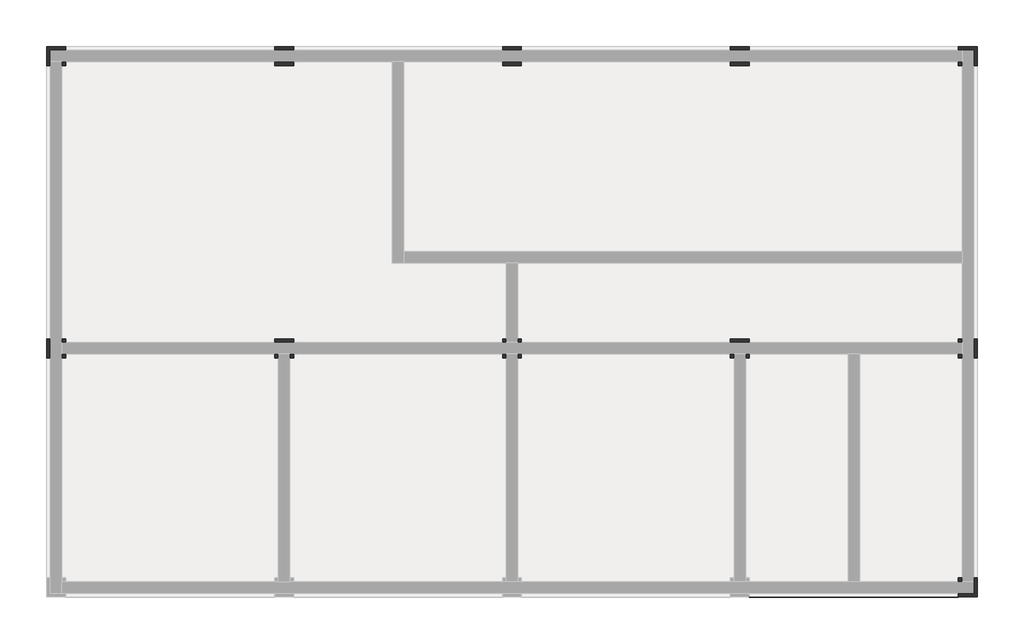
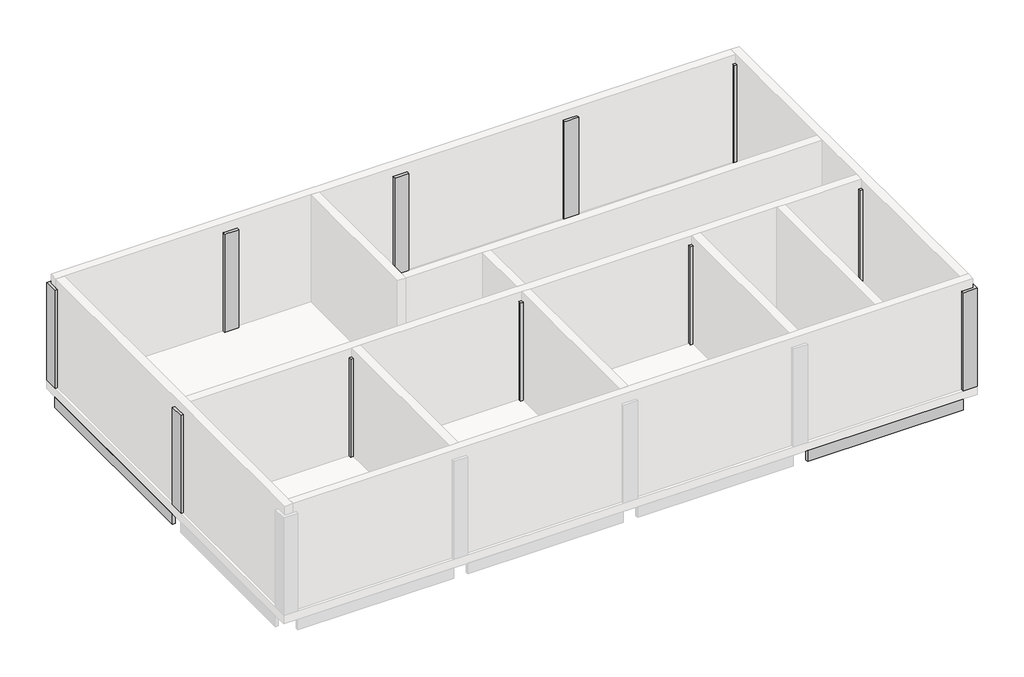
# One storey, part 2 of 2: 15 beams, 11 columns.
"""IFC4 building model written with IfcOpenShell, lengths in millimetres."""

from ifc_helpers import new_model, si_unit, frame, origin, place, context, project, spatial, polyline, outline, extrude, faceted_brep, element, save

model = new_model("IFC4")

# Units and contexts
model_context = context("Model", 3, world=origin())
ifc_project = project(units=[si_unit("LENGTHUNIT", "METRE", prefix="MILLI")], contexts=[model_context])

# Site, building, storey
site = spatial("IfcSite", under=ifc_project)
building = spatial("IfcBuilding", under=site)
storey = spatial("IfcBuildingStorey", under=building, Name="2nd FL GL+6,200", Elevation=6000.0)

# Beams
placement = place(None, origin())
element("IfcBeam", 1, ObjectType="RC Beam_Rectangular : 350 x 700mm", at=placement, inside=storey, context=model_context, shape_type="SweptSolid", body=[
    extrude(outline(polyline([(-18945.7273237, 9185.9763125), (-18845.7273237, 9185.9763125), (-18845.7273237, 1985.9763125), (-18945.7273237, 1985.9763125), (-18945.7273237, 9185.9763125)])), frame((0.0, 0.0, 5300.0), z_axis=(0.0, 0.0, 1.0), x_axis=(1.0, 0.0, 0.0)), (0.0, 0.0, 1.0), 400.0),
])
element("IfcBeam", 2, ObjectType="RC Beam_Rectangular : 350 x 700mm", at=placement, inside=storey, context=model_context, shape_type="SweptSolid", body=[
    extrude(outline(polyline([(-12870.7273237, 9185.9763125), (-12520.7273237, 9185.9763125), (-12520.7273237, 1985.9763125), (-12870.7273237, 1985.9763125), (-12870.7273237, 9185.9763125)])), frame((0.0, 0.0, 5300.0), z_axis=(0.0, 0.0, 1.0), x_axis=(1.0, 0.0, 0.0)), (0.0, 0.0, 1.0), 400.0),
])
element("IfcBeam", 3, ObjectType="RC Beam_Rectangular : 350 x 700mm", at=placement, inside=storey, context=model_context, shape_type="SweptSolid", body=[
    extrude(outline(polyline([(-6870.7273237, 9185.9763125), (-6520.7273237, 9185.9763125), (-6520.7273237, 1985.9763125), (-6870.7273237, 1985.9763125), (-6870.7273237, 9185.9763125)])), frame((0.0, 0.0, 5300.0), z_axis=(0.0, 0.0, 1.0), x_axis=(1.0, 0.0, 0.0)), (0.0, 0.0, 1.0), 400.0),
])
element("IfcBeam", 4, ObjectType="RC Beam_Rectangular : 350 x 700mm", at=placement, inside=storey, context=model_context, shape_type="SweptSolid", body=[
    extrude(outline(polyline([(-870.7273237, 9185.9763125), (-520.7273237, 9185.9763125), (-520.7273237, 1985.9763125), (-870.7273237, 1985.9763125), (-870.7273237, 9185.9763125)])), frame((0.0, 0.0, 5300.0), z_axis=(0.0, 0.0, 1.0), x_axis=(1.0, 0.0, 0.0)), (0.0, 0.0, 1.0), 400.0),
])
element("IfcBeam", 5, ObjectType="RC Beam_Rectangular : 350 x 700mm", at=placement, inside=storey, context=model_context, shape_type="SweptSolid", body=[
    extrude(outline(polyline([(5554.2726763, 1485.9763125), (5554.2726763, -4314.0236875), (5454.2726763, -4314.0236875), (5454.2726763, 1485.9763125), (5554.2726763, 1485.9763125)])), frame((0.0, 0.0, 5300.0), z_axis=(0.0, 0.0, 1.0), x_axis=(1.0, 0.0, 0.0)), (0.0, 0.0, 1.0), 400.0),
])
element("IfcBeam", 6, ObjectType="RC Beam_Rectangular : 350 x 700mm", at=placement, inside=storey, context=model_context, shape_type="SweptSolid", body=[
    extrude(outline(polyline([(5554.2726763, 9185.9763125), (5554.2726763, 1998.6763125), (5454.2726763, 1998.6763125), (5454.2726763, 9185.9763125), (5554.2726763, 9185.9763125)])), frame((0.0, 0.0, 5300.0), z_axis=(0.0, 0.0, 1.0), x_axis=(1.0, 0.0, 0.0)), (0.0, 0.0, 1.0), 400.0),
])
element("IfcBeam", 7, ObjectType="RC Beam_Rectangular : 350 x 700mm", at=placement, inside=storey, context=model_context, shape_type="SweptSolid", body=[
    extrude(outline(polyline([(-18445.7273237, 9685.9763125), (-12945.7273237, 9685.9763125), (-12945.7273237, 9585.9763125), (-18445.7273237, 9585.9763125), (-18445.7273237, 9685.9763125)])), frame((0.0, 0.0, 5300.0), z_axis=(0.0, 0.0, 1.0), x_axis=(1.0, 0.0, 0.0)), (0.0, 0.0, 1.0), 400.0),
])
element("IfcBeam", 8, ObjectType="RC Beam_Rectangular : 350 x 700mm", at=placement, inside=storey, context=model_context, shape_type="SweptSolid", body=[
    extrude(outline(polyline([(-12433.0273237, 9685.9763125), (-6945.7273237, 9685.9763125), (-6945.7273237, 9585.9763125), (-12433.0273237, 9585.9763125), (-12433.0273237, 9685.9763125)])), frame((0.0, 0.0, 5300.0), z_axis=(0.0, 0.0, 1.0), x_axis=(1.0, 0.0, 0.0)), (0.0, 0.0, 1.0), 400.0),
])
element("IfcBeam", 9, ObjectType="RC Beam_Rectangular : 350 x 700mm", at=placement, inside=storey, context=model_context, shape_type="SweptSolid", body=[
    extrude(outline(polyline([(-6433.0273237, 9685.9763125), (-945.7273237, 9685.9763125), (-945.7273237, 9585.9763125), (-6433.0273237, 9585.9763125), (-6433.0273237, 9685.9763125)])), frame((0.0, 0.0, 5300.0), z_axis=(0.0, 0.0, 1.0), x_axis=(1.0, 0.0, 0.0)), (0.0, 0.0, 1.0), 400.0),
])
element("IfcBeam", 10, ObjectType="RC Beam_Rectangular : 350 x 700mm", at=placement, inside=storey, context=model_context, shape_type="SweptSolid", body=[
    extrude(outline(polyline([(-433.0273237, 9685.9763125), (5054.2726763, 9685.9763125), (5054.2726763, 9585.9763125), (-433.0273237, 9585.9763125), (-433.0273237, 9685.9763125)])), frame((0.0, 0.0, 5300.0), z_axis=(0.0, 0.0, 1.0), x_axis=(1.0, 0.0, 0.0)), (0.0, 0.0, 1.0), 400.0),
])
element("IfcBeam", 11, ObjectType="RC Beam_Rectangular : 350 x 700mm", at=placement, inside=storey, context=model_context, shape_type="SweptSolid", body=[
    extrude(outline(polyline([(-12945.7273237, 1560.9763125), (-18445.7273237, 1560.9763125), (-18445.7273237, 1585.9763125), (-12945.7273237, 1585.9763125), (-12945.7273237, 1560.9763125)])), frame((0.0, 0.0, 5300.0), z_axis=(0.0, 0.0, 1.0), x_axis=(1.0, 0.0, 0.0)), (0.0, 0.0, 1.0), 400.0),
    extrude(outline(polyline([(-18445.7273237, 1910.9763125), (-12945.7273237, 1910.9763125), (-12945.7273237, 1885.9763125), (-18445.7273237, 1885.9763125), (-18445.7273237, 1910.9763125)])), frame((0.0, 0.0, 5300.0), z_axis=(0.0, 0.0, 1.0), x_axis=(1.0, 0.0, 0.0)), (0.0, 0.0, 1.0), 400.0),
])
element("IfcBeam", 12, ObjectType="RC Beam_Rectangular : 350 x 700mm", at=placement, inside=storey, context=model_context, shape_type="SweptSolid", body=[
    extrude(outline(polyline([(-6945.7273237, 1585.9763125), (-6945.7273237, 1560.9763125), (-12445.7273237, 1560.9763125), (-12445.7273237, 1585.9763125), (-6945.7273237, 1585.9763125)])), frame((0.0, 0.0, 5300.0), z_axis=(0.0, 0.0, 1.0), x_axis=(1.0, 0.0, 0.0)), (0.0, 0.0, 1.0), 400.0),
    extrude(outline(polyline([(-6945.7273237, 1910.9763125), (-6945.7273237, 1885.9763125), (-12445.7273237, 1885.9763125), (-12445.7273237, 1910.9763125), (-6945.7273237, 1910.9763125)])), frame((0.0, 0.0, 5300.0), z_axis=(0.0, 0.0, 1.0), x_axis=(1.0, 0.0, 0.0)), (0.0, 0.0, 1.0), 400.0),
])
element("IfcBeam", 13, ObjectType="RC Beam_Rectangular : 350 x 700mm", at=placement, inside=storey, context=model_context, shape_type="SweptSolid", body=[
    extrude(outline(polyline([(-945.7273237, 1585.9763125), (-945.7273237, 1560.9763125), (-6445.7273237, 1560.9763125), (-6445.7273237, 1585.9763125), (-945.7273237, 1585.9763125)])), frame((0.0, 0.0, 5300.0), z_axis=(0.0, 0.0, 1.0), x_axis=(1.0, 0.0, 0.0)), (0.0, 0.0, 1.0), 400.0),
    extrude(outline(polyline([(-945.7273237, 1910.9763125), (-945.7273237, 1885.9763125), (-6445.7273237, 1885.9763125), (-6445.7273237, 1910.9763125), (-945.7273237, 1910.9763125)])), frame((0.0, 0.0, 5300.0), z_axis=(0.0, 0.0, 1.0), x_axis=(1.0, 0.0, 0.0)), (0.0, 0.0, 1.0), 400.0),
])
element("IfcBeam", 14, ObjectType="RC Beam_Rectangular : 350 x 700mm", at=placement, inside=storey, context=model_context, shape_type="SweptSolid", body=[
    extrude(outline(polyline([(2154.2726763, 1585.9763125), (2154.2726763, 1560.9763125), (-445.7273237, 1560.9763125), (-445.7273237, 1585.9763125), (2154.2726763, 1585.9763125)])), frame((0.0, 0.0, 5300.0), z_axis=(0.0, 0.0, 1.0), x_axis=(1.0, 0.0, 0.0)), (0.0, 0.0, 1.0), 400.0),
    extrude(outline(polyline([(5054.2726763, 1910.9763125), (5054.2726763, 1885.9763125), (-445.7273237, 1885.9763125), (-445.7273237, 1910.9763125), (5054.2726763, 1910.9763125)])), frame((0.0, 0.0, 5300.0), z_axis=(0.0, 0.0, 1.0), x_axis=(1.0, 0.0, 0.0)), (0.0, 0.0, 1.0), 400.0),
    extrude(outline(polyline([(5054.2726763, 1585.9763125), (5054.2726763, 1560.9763125), (2454.2726763, 1560.9763125), (2454.2726763, 1585.9763125), (5054.2726763, 1585.9763125)])), frame((0.0, 0.0, 5300.0), z_axis=(0.0, 0.0, 1.0), x_axis=(1.0, 0.0, 0.0)), (0.0, 0.0, 1.0), 400.0),
])
element("IfcBeam", 15, ObjectType="RC Beam_Rectangular : 350 x 700mm", at=placement, inside=storey, context=model_context, shape_type="SweptSolid", body=[
    extrude(outline(polyline([(5054.2726763, -4714.0236875), (5054.2726763, -4814.0236875), (-445.7273237, -4814.0236875), (-445.7273237, -4714.0236875), (5054.2726763, -4714.0236875)])), frame((0.0, 0.0, 5300.0), z_axis=(0.0, 0.0, 1.0), x_axis=(1.0, 0.0, 0.0)), (0.0, 0.0, 1.0), 400.0),
])

# Columns
element("IfcColumn", 16, ObjectType="RC_Column_Rectangular : 500 x 500mm", at=placement, inside=storey, context=model_context, shape_type="Brep", body=[
    faceted_brep([(-18945.7273237, 9185.9763125, 6000.0), (-18945.7273237, 9685.9763125, 6000.0), (-18445.7273237, 9685.9763125, 6000.0), (-18445.7273237, 9585.9763125, 6000.0), (-18845.7273237, 9585.9763125, 6000.0), (-18845.7273237, 9285.9763125, 6000.0), (-18845.7273237, 9185.9763125, 6000.0), (-18945.7273237, 9685.9763125, 9667.0), (-18445.7273237, 9685.9763125, 9667.0), (-18445.7273237, 9685.9763125, 9300.0), (-18945.7273237, 9185.9763125, 9300.0), (-18945.7273237, 9185.9763125, 9667.0), (-18845.7273237, 9185.9763125, 9300.0), (-18845.7273237, 9185.9763125, 9667.0), (-18445.7273237, 9585.9763125, 9667.0), (-18445.7273237, 9585.9763125, 9300.0), (-18845.7273237, 9585.9763125, 9667.0)], [[[0, 1, 2, 3, 4, 5, 6]], [[2, 1, 7, 8, 9]], [[1, 0, 10, 11, 7]], [[11, 10, 0, 6, 12, 13]], [[2, 9, 8, 14, 15, 3]], [[8, 7, 11, 13, 16, 14]], [[16, 4, 3, 15, 14]], [[4, 16, 13, 12, 6, 5]]]),
    faceted_brep([(-18445.7273237, 9285.9763125, 9667.0), (-18445.7273237, 9285.9763125, 6000.0), (-18545.7273237, 9285.9763125, 6000.0), (-18545.7273237, 9285.9763125, 9667.0), (-18445.7273237, 9185.9763125, 9667.0), (-18445.7273237, 9185.9763125, 6000.0), (-18545.7273237, 9185.9763125, 6000.0), (-18545.7273237, 9185.9763125, 9667.0)], [[[0, 1, 2, 3]], [[4, 5, 1, 0]], [[2, 6, 7, 3]], [[1, 5, 6, 2]], [[5, 4, 7, 6]], [[4, 0, 3, 7]]]),
])
element("IfcColumn", 17, ObjectType="RC_Column_Rectangular : 500 x 500mm", at=placement, inside=storey, context=model_context, shape_type="Brep", body=[
    faceted_brep([(-18945.7273237, 1485.9763125, 6000.0), (-18945.7273237, 1985.9763125, 6000.0), (-18845.7273237, 1985.9763125, 6000.0), (-18845.7273237, 1485.9763125, 6000.0), (-18945.7273237, 1485.9763125, 9300.0), (-18945.7273237, 1485.9763125, 9667.0), (-18945.7273237, 1985.9763125, 9667.0), (-18845.7273237, 1485.9763125, 9300.0), (-18845.7273237, 1485.9763125, 9667.0), (-18845.7273237, 1985.9763125, 9667.0)], [[[0, 1, 2, 3]], [[1, 0, 4, 5, 6]], [[5, 4, 0, 3, 7, 8]], [[6, 5, 8, 9]], [[3, 2, 9, 8, 7]], [[1, 6, 9, 2]]]),
    faceted_brep([(-18445.7273237, 1985.9763125, 9667.0), (-18445.7273237, 1985.9763125, 6000.0), (-18545.7273237, 1985.9763125, 6000.0), (-18545.7273237, 1985.9763125, 9667.0), (-18445.7273237, 1910.9763125, 9667.0), (-18445.7273237, 1885.9763125, 9667.0), (-18445.7273237, 1885.9763125, 9300.0), (-18445.7273237, 1885.9763125, 6000.0), (-18545.7273237, 1885.9763125, 6000.0), (-18545.7273237, 1885.9763125, 9667.0)], [[[0, 1, 2, 3]], [[1, 0, 4, 5, 6, 7]], [[2, 1, 7, 8]], [[0, 3, 9, 5, 4]], [[7, 6, 5, 9, 8]], [[3, 2, 8, 9]]]),
    faceted_brep([(-18545.7273237, 1485.9763125, 6000.0), (-18545.7273237, 1485.9763125, 9667.0), (-18545.7273237, 1585.9763125, 9667.0), (-18545.7273237, 1585.9763125, 6000.0), (-18445.7273237, 1485.9763125, 6000.0), (-18445.7273237, 1485.9763125, 9667.0), (-18445.7273237, 1585.9763125, 9667.0), (-18445.7273237, 1585.9763125, 9300.0), (-18445.7273237, 1585.9763125, 6000.0), (-18445.7273237, 1560.9763125, 9667.0)], [[[0, 1, 2, 3]], [[4, 5, 1, 0]], [[6, 7, 8, 3, 2]], [[5, 4, 8, 7, 6, 9]], [[4, 0, 3, 8]], [[1, 5, 9, 6, 2]]]),
])
element("IfcColumn", 18, ObjectType="RC_Column_Rectangular : 500 x 500mm", at=placement, inside=storey, context=model_context, shape_type="Brep", body=[
    faceted_brep([(-12945.7273237, 9685.9763125, 6000.0), (-12445.7273237, 9685.9763125, 6000.0), (-12445.7273237, 9585.9763125, 6000.0), (-12945.7273237, 9585.9763125, 6000.0), (-12945.7273237, 9685.9763125, 9300.0), (-12945.7273237, 9685.9763125, 9667.0), (-12445.7273237, 9685.9763125, 9667.0), (-12445.7273237, 9685.9763125, 9300.0), (-12945.7273237, 9585.9763125, 9300.0), (-12945.7273237, 9585.9763125, 9667.0), (-12445.7273237, 9585.9763125, 9667.0), (-12445.7273237, 9585.9763125, 9300.0)], [[[0, 1, 2, 3]], [[1, 0, 4, 5, 6, 7]], [[5, 4, 0, 3, 8, 9]], [[1, 7, 6, 10, 11, 2]], [[6, 5, 9, 10]], [[3, 2, 11, 10, 9, 8]]]),
    faceted_brep([(-12945.7273237, 9185.9763125, 6000.0), (-12445.7273237, 9185.9763125, 6000.0), (-12445.7273237, 9185.9763125, 9667.0), (-12520.7273237, 9185.9763125, 9667.0), (-12870.7273237, 9185.9763125, 9667.0), (-12945.7273237, 9185.9763125, 9667.0), (-12445.7273237, 9285.9763125, 6000.0), (-12945.7273237, 9285.9763125, 6000.0), (-12945.7273237, 9285.9763125, 9667.0), (-12445.7273237, 9285.9763125, 9667.0)], [[[0, 1, 2, 3, 4, 5]], [[6, 7, 8, 9]], [[1, 0, 7, 6]], [[0, 5, 8, 7]], [[2, 1, 6, 9]], [[5, 4, 3, 2, 9, 8]]]),
])
element("IfcColumn", 19, ObjectType="RC_Column_Rectangular : 500 x 500mm", at=placement, inside=storey, context=model_context, shape_type="Brep", body=[
    faceted_brep([(-12945.7273237, 1985.9763125, 6000.0), (-12445.7273237, 1985.9763125, 6000.0), (-12445.7273237, 1885.9763125, 6000.0), (-12945.7273237, 1885.9763125, 6000.0), (-12945.7273237, 1985.9763125, 9667.0), (-12870.7273237, 1985.9763125, 9667.0), (-12520.7273237, 1985.9763125, 9667.0), (-12445.7273237, 1985.9763125, 9667.0), (-12945.7273237, 1885.9763125, 9300.0), (-12945.7273237, 1885.9763125, 9667.0), (-12945.7273237, 1910.9763125, 9667.0), (-12445.7273237, 1910.9763125, 9667.0), (-12445.7273237, 1885.9763125, 9667.0), (-12445.7273237, 1885.9763125, 9300.0)], [[[0, 1, 2, 3]], [[1, 0, 4, 5, 6, 7]], [[4, 0, 3, 8, 9, 10]], [[1, 7, 11, 12, 13, 2]], [[7, 6, 5, 4, 10, 9, 12, 11]], [[3, 2, 13, 12, 9, 8]]]),
    faceted_brep([(-12945.7273237, 1485.9763125, 9667.0), (-12945.7273237, 1485.9763125, 6000.0), (-12845.7273237, 1485.9763125, 6000.0), (-12845.7273237, 1485.9763125, 9300.0), (-12845.7273237, 1485.9763125, 9667.0), (-12870.7273237, 1485.9763125, 9667.0), (-12945.7273237, 1585.9763125, 6000.0), (-12945.7273237, 1585.9763125, 9300.0), (-12945.7273237, 1585.9763125, 9667.0), (-12845.7273237, 1585.9763125, 9667.0), (-12845.7273237, 1585.9763125, 6000.0), (-12945.7273237, 1560.9763125, 9667.0)], [[[0, 1, 2, 3, 4, 5]], [[6, 7, 8, 9, 10]], [[1, 6, 10, 2]], [[1, 0, 11, 8, 7, 6]], [[8, 11, 0, 5, 4, 9]], [[4, 3, 2, 10, 9]]]),
    faceted_brep([(-12445.7273237, 1485.9763125, 9667.0), (-12445.7273237, 1485.9763125, 6000.0), (-12445.7273237, 1585.9763125, 6000.0), (-12445.7273237, 1585.9763125, 9300.0), (-12445.7273237, 1585.9763125, 9667.0), (-12445.7273237, 1560.9763125, 9667.0), (-12545.7273237, 1485.9763125, 6000.0), (-12545.7273237, 1485.9763125, 9300.0), (-12545.7273237, 1485.9763125, 9667.0), (-12545.7273237, 1585.9763125, 9667.0), (-12545.7273237, 1585.9763125, 6000.0), (-12520.7273237, 1485.9763125, 9667.0)], [[[0, 1, 2, 3, 4, 5]], [[6, 7, 8, 9, 10]], [[1, 0, 11, 8, 7, 6]], [[4, 3, 2, 10, 9]], [[2, 1, 6, 10]], [[0, 5, 4, 9, 8, 11]]]),
])
element("IfcColumn", 20, ObjectType="RC_Column_Rectangular : 500 x 500mm", at=placement, inside=storey, context=model_context, shape_type="Brep", body=[
    faceted_brep([(-6945.7273237, 9685.9763125, 6000.0), (-6445.7273237, 9685.9763125, 6000.0), (-6445.7273237, 9585.9763125, 6000.0), (-6945.7273237, 9585.9763125, 6000.0), (-6945.7273237, 9685.9763125, 9300.0), (-6945.7273237, 9685.9763125, 9667.0), (-6445.7273237, 9685.9763125, 9667.0), (-6445.7273237, 9685.9763125, 9300.0), (-6945.7273237, 9585.9763125, 9300.0), (-6945.7273237, 9585.9763125, 9667.0), (-6445.7273237, 9585.9763125, 9667.0), (-6445.7273237, 9585.9763125, 9300.0)], [[[0, 1, 2, 3]], [[1, 0, 4, 5, 6, 7]], [[5, 4, 0, 3, 8, 9]], [[1, 7, 6, 10, 11, 2]], [[6, 5, 9, 10]], [[3, 2, 11, 10, 9, 8]]]),
    faceted_brep([(-6945.7273237, 9185.9763125, 6000.0), (-6445.7273237, 9185.9763125, 6000.0), (-6445.7273237, 9185.9763125, 9667.0), (-6520.7273237, 9185.9763125, 9667.0), (-6870.7273237, 9185.9763125, 9667.0), (-6945.7273237, 9185.9763125, 9667.0), (-6445.7273237, 9285.9763125, 6000.0), (-6945.7273237, 9285.9763125, 6000.0), (-6945.7273237, 9285.9763125, 9667.0), (-6445.7273237, 9285.9763125, 9667.0)], [[[0, 1, 2, 3, 4, 5]], [[6, 7, 8, 9]], [[1, 0, 7, 6]], [[0, 5, 8, 7]], [[2, 1, 6, 9]], [[5, 4, 3, 2, 9, 8]]]),
])
element("IfcColumn", 21, ObjectType="RC_Column_Rectangular : 500 x 500mm", at=placement, inside=storey, context=model_context, shape_type="Brep", body=[
    faceted_brep([(-6945.7273237, 1885.9763125, 6000.0), (-6945.7273237, 1985.9763125, 6000.0), (-6845.7273237, 1985.9763125, 6000.0), (-6845.7273237, 1885.9763125, 6000.0), (-6945.7273237, 1985.9763125, 9667.0), (-6945.7273237, 1885.9763125, 9300.0), (-6945.7273237, 1885.9763125, 9667.0), (-6945.7273237, 1910.9763125, 9667.0), (-6845.7273237, 1885.9763125, 9667.0), (-6845.7273237, 1985.9763125, 9667.0), (-6870.7273237, 1985.9763125, 9667.0), (-6845.7273237, 1985.9763125, 9300.0)], [[[0, 1, 2, 3]], [[4, 1, 0, 5, 6, 7]], [[4, 7, 6, 8, 9, 10]], [[3, 2, 11, 9, 8]], [[1, 4, 10, 9, 11, 2]], [[6, 5, 0, 3, 8]]]),
    faceted_brep([(-6445.7273237, 1985.9763125, 9667.0), (-6445.7273237, 1985.9763125, 6000.0), (-6545.7273237, 1985.9763125, 6000.0), (-6545.7273237, 1985.9763125, 9300.0), (-6545.7273237, 1985.9763125, 9667.0), (-6520.7273237, 1985.9763125, 9667.0), (-6445.7273237, 1910.9763125, 9667.0), (-6445.7273237, 1885.9763125, 9667.0), (-6445.7273237, 1885.9763125, 9300.0), (-6445.7273237, 1885.9763125, 6000.0), (-6545.7273237, 1885.9763125, 9667.0), (-6545.7273237, 1885.9763125, 6000.0)], [[[0, 1, 2, 3, 4, 5]], [[1, 0, 6, 7, 8, 9]], [[9, 8, 7, 10, 11]], [[2, 11, 10, 4, 3]], [[1, 9, 11, 2]], [[7, 6, 0, 5, 4, 10]]]),
    faceted_brep([(-6945.7273237, 1485.9763125, 9667.0), (-6945.7273237, 1485.9763125, 6000.0), (-6845.7273237, 1485.9763125, 6000.0), (-6845.7273237, 1485.9763125, 9300.0), (-6845.7273237, 1485.9763125, 9667.0), (-6870.7273237, 1485.9763125, 9667.0), (-6945.7273237, 1585.9763125, 6000.0), (-6945.7273237, 1585.9763125, 9300.0), (-6945.7273237, 1585.9763125, 9667.0), (-6845.7273237, 1585.9763125, 9667.0), (-6845.7273237, 1585.9763125, 6000.0), (-6945.7273237, 1560.9763125, 9667.0)], [[[0, 1, 2, 3, 4, 5]], [[6, 7, 8, 9, 10]], [[1, 6, 10, 2]], [[1, 0, 11, 8, 7, 6]], [[8, 11, 0, 5, 4, 9]], [[4, 3, 2, 10, 9]]]),
    faceted_brep([(-6445.7273237, 1485.9763125, 9667.0), (-6445.7273237, 1485.9763125, 6000.0), (-6445.7273237, 1585.9763125, 6000.0), (-6445.7273237, 1585.9763125, 9300.0), (-6445.7273237, 1585.9763125, 9667.0), (-6445.7273237, 1560.9763125, 9667.0), (-6545.7273237, 1485.9763125, 6000.0), (-6545.7273237, 1485.9763125, 9300.0), (-6545.7273237, 1485.9763125, 9667.0), (-6545.7273237, 1585.9763125, 9667.0), (-6545.7273237, 1585.9763125, 6000.0), (-6520.7273237, 1485.9763125, 9667.0)], [[[0, 1, 2, 3, 4, 5]], [[6, 7, 8, 9, 10]], [[1, 0, 11, 8, 7, 6]], [[4, 3, 2, 10, 9]], [[2, 1, 6, 10]], [[0, 5, 4, 9, 8, 11]]]),
])
element("IfcColumn", 22, ObjectType="RC_Column_Rectangular : 500 x 500mm", at=placement, inside=storey, context=model_context, shape_type="Brep", body=[
    faceted_brep([(-945.7273237, 9685.9763125, 6000.0), (-445.7273237, 9685.9763125, 6000.0), (-445.7273237, 9585.9763125, 6000.0), (-945.7273237, 9585.9763125, 6000.0), (-945.7273237, 9685.9763125, 9300.0), (-945.7273237, 9685.9763125, 9667.0), (-445.7273237, 9685.9763125, 9667.0), (-445.7273237, 9685.9763125, 9300.0), (-945.7273237, 9585.9763125, 9300.0), (-945.7273237, 9585.9763125, 9667.0), (-445.7273237, 9585.9763125, 9667.0), (-445.7273237, 9585.9763125, 9300.0)], [[[0, 1, 2, 3]], [[1, 0, 4, 5, 6, 7]], [[5, 4, 0, 3, 8, 9]], [[1, 7, 6, 10, 11, 2]], [[6, 5, 9, 10]], [[3, 2, 11, 10, 9, 8]]]),
    faceted_brep([(-945.7273237, 9185.9763125, 6000.0), (-445.7273237, 9185.9763125, 6000.0), (-445.7273237, 9185.9763125, 9667.0), (-520.7273237, 9185.9763125, 9667.0), (-870.7273237, 9185.9763125, 9667.0), (-945.7273237, 9185.9763125, 9667.0), (-445.7273237, 9285.9763125, 6000.0), (-945.7273237, 9285.9763125, 6000.0), (-945.7273237, 9285.9763125, 9667.0), (-445.7273237, 9285.9763125, 9667.0)], [[[0, 1, 2, 3, 4, 5]], [[6, 7, 8, 9]], [[1, 0, 7, 6]], [[0, 5, 8, 7]], [[2, 1, 6, 9]], [[5, 4, 3, 2, 9, 8]]]),
])
element("IfcColumn", 23, ObjectType="RC_Column_Rectangular : 500 x 500mm", at=placement, inside=storey, context=model_context, shape_type="Brep", body=[
    faceted_brep([(-945.7273237, 1985.9763125, 6000.0), (-445.7273237, 1985.9763125, 6000.0), (-445.7273237, 1885.9763125, 6000.0), (-945.7273237, 1885.9763125, 6000.0), (-945.7273237, 1985.9763125, 9667.0), (-870.7273237, 1985.9763125, 9667.0), (-520.7273237, 1985.9763125, 9667.0), (-445.7273237, 1985.9763125, 9667.0), (-945.7273237, 1885.9763125, 9300.0), (-945.7273237, 1885.9763125, 9667.0), (-945.7273237, 1910.9763125, 9667.0), (-445.7273237, 1910.9763125, 9667.0), (-445.7273237, 1885.9763125, 9667.0), (-445.7273237, 1885.9763125, 9300.0)], [[[0, 1, 2, 3]], [[1, 0, 4, 5, 6, 7]], [[4, 0, 3, 8, 9, 10]], [[1, 7, 11, 12, 13, 2]], [[7, 6, 5, 4, 10, 9, 12, 11]], [[3, 2, 13, 12, 9, 8]]]),
    faceted_brep([(-945.7273237, 1485.9763125, 9667.0), (-945.7273237, 1485.9763125, 6000.0), (-845.7273237, 1485.9763125, 6000.0), (-845.7273237, 1485.9763125, 9300.0), (-845.7273237, 1485.9763125, 9667.0), (-870.7273237, 1485.9763125, 9667.0), (-945.7273237, 1585.9763125, 6000.0), (-945.7273237, 1585.9763125, 9300.0), (-945.7273237, 1585.9763125, 9667.0), (-845.7273237, 1585.9763125, 9667.0), (-845.7273237, 1585.9763125, 6000.0), (-945.7273237, 1560.9763125, 9667.0)], [[[0, 1, 2, 3, 4, 5]], [[6, 7, 8, 9, 10]], [[1, 6, 10, 2]], [[1, 0, 11, 8, 7, 6]], [[8, 11, 0, 5, 4, 9]], [[4, 3, 2, 10, 9]]]),
    faceted_brep([(-445.7273237, 1485.9763125, 9667.0), (-445.7273237, 1485.9763125, 6000.0), (-445.7273237, 1585.9763125, 6000.0), (-445.7273237, 1585.9763125, 9300.0), (-445.7273237, 1585.9763125, 9667.0), (-445.7273237, 1560.9763125, 9667.0), (-545.7273237, 1485.9763125, 6000.0), (-545.7273237, 1485.9763125, 9300.0), (-545.7273237, 1485.9763125, 9667.0), (-545.7273237, 1585.9763125, 9667.0), (-545.7273237, 1585.9763125, 6000.0), (-520.7273237, 1485.9763125, 9667.0)], [[[0, 1, 2, 3, 4, 5]], [[6, 7, 8, 9, 10]], [[1, 0, 11, 8, 7, 6]], [[4, 3, 2, 10, 9]], [[2, 1, 6, 10]], [[0, 5, 4, 9, 8, 11]]]),
])
element("IfcColumn", 24, ObjectType="RC_Column_Rectangular : 500 x 500mm", at=placement, inside=storey, context=model_context, shape_type="Brep", body=[
    faceted_brep([(5054.2726763, 9185.9763125, 6000.0), (5054.2726763, 9285.9763125, 6000.0), (5154.2726763, 9285.9763125, 6000.0), (5154.2726763, 9185.9763125, 6000.0), (5054.2726763, 9185.9763125, 9667.0), (5154.2726763, 9185.9763125, 9667.0), (5054.2726763, 9285.9763125, 9667.0), (5154.2726763, 9285.9763125, 9667.0)], [[[0, 1, 2, 3]], [[4, 0, 3, 5]], [[6, 4, 5, 7]], [[2, 1, 6, 7]], [[0, 4, 6, 1]], [[3, 2, 7, 5]]]),
    faceted_brep([(5554.2726763, 9685.9763125, 6000.0), (5054.2726763, 9685.9763125, 6000.0), (5054.2726763, 9685.9763125, 9300.0), (5054.2726763, 9685.9763125, 9667.0), (5554.2726763, 9685.9763125, 9667.0), (5054.2726763, 9585.9763125, 6000.0), (5054.2726763, 9585.9763125, 9300.0), (5054.2726763, 9585.9763125, 9667.0), (5554.2726763, 9185.9763125, 6000.0), (5554.2726763, 9185.9763125, 9667.0), (5554.2726763, 9185.9763125, 9300.0), (5454.2726763, 9585.9763125, 6000.0), (5454.2726763, 9585.9763125, 9667.0), (5154.2726763, 9585.9763125, 6000.0), (5454.2726763, 9185.9763125, 6000.0), (5454.2726763, 9185.9763125, 9300.0), (5454.2726763, 9185.9763125, 9667.0)], [[[0, 1, 2, 3, 4]], [[3, 2, 1, 5, 6, 7]], [[8, 0, 4, 9, 10]], [[11, 12, 7, 6, 5, 13]], [[12, 11, 14, 15, 16]], [[0, 8, 14, 11, 13, 5, 1]], [[8, 10, 9, 16, 15, 14]], [[4, 3, 7, 12, 16, 9]]]),
])
element("IfcColumn", 25, ObjectType="RC_Column_Rectangular : 500 x 500mm", at=placement, inside=storey, context=model_context, shape_type="Brep", body=[
    faceted_brep([(5054.2726763, 1985.9763125, 6000.0), (5154.2726763, 1985.9763125, 6000.0), (5154.2726763, 1885.9763125, 6000.0), (5054.2726763, 1885.9763125, 6000.0), (5054.2726763, 1985.9763125, 9667.0), (5054.2726763, 1885.9763125, 9300.0), (5054.2726763, 1885.9763125, 9667.0), (5054.2726763, 1910.9763125, 9667.0), (5154.2726763, 1985.9763125, 9667.0), (5154.2726763, 1885.9763125, 9667.0)], [[[0, 1, 2, 3]], [[4, 0, 3, 5, 6, 7]], [[1, 8, 9, 2]], [[0, 4, 8, 1]], [[3, 2, 9, 6, 5]], [[8, 4, 7, 6, 9]]]),
    faceted_brep([(5554.2726763, 1985.9763125, 9667.0), (5554.2726763, 1985.9763125, 6000.0), (5454.2726763, 1985.9763125, 6000.0), (5454.2726763, 1985.9763125, 9667.0), (5554.2726763, 1485.9763125, 6000.0), (5554.2726763, 1485.9763125, 9667.0), (5554.2726763, 1485.9763125, 9300.0), (5454.2726763, 1485.9763125, 6000.0), (5454.2726763, 1485.9763125, 9300.0), (5454.2726763, 1485.9763125, 9667.0)], [[[0, 1, 2, 3]], [[4, 1, 0, 5, 6]], [[2, 7, 8, 9, 3]], [[1, 4, 7, 2]], [[4, 6, 5, 9, 8, 7]], [[5, 0, 3, 9]]]),
    faceted_brep([(5054.2726763, 1485.9763125, 9667.0), (5054.2726763, 1485.9763125, 6000.0), (5154.2726763, 1485.9763125, 6000.0), (5154.2726763, 1485.9763125, 9667.0), (5154.2726763, 1585.9763125, 9667.0), (5054.2726763, 1585.9763125, 9667.0), (5054.2726763, 1560.9763125, 9667.0), (5154.2726763, 1585.9763125, 6000.0), (5054.2726763, 1585.9763125, 6000.0), (5054.2726763, 1585.9763125, 9300.0)], [[[0, 1, 2, 3]], [[0, 3, 4, 5, 6]], [[7, 8, 9, 5, 4]], [[2, 1, 8, 7]], [[1, 0, 6, 5, 9, 8]], [[3, 2, 7, 4]]]),
])
element("IfcColumn", 26, ObjectType="RC_Column_Rectangular : 500 x 500mm", at=placement, inside=storey, context=model_context, shape_type="Brep", body=[
    faceted_brep([(5054.2726763, -4414.0236875, 6000.0), (5054.2726763, -4314.0236875, 6000.0), (5154.2726763, -4314.0236875, 6000.0), (5154.2726763, -4414.0236875, 6000.0), (5054.2726763, -4314.0236875, 9667.0), (5054.2726763, -4414.0236875, 9667.0), (5154.2726763, -4414.0236875, 9667.0), (5154.2726763, -4314.0236875, 9667.0)], [[[0, 1, 2, 3]], [[4, 1, 0, 5]], [[4, 5, 6, 7]], [[5, 0, 3, 6]], [[3, 2, 7, 6]], [[1, 4, 7, 2]]]),
    faceted_brep([(5554.2726763, -4314.0236875, 9667.0), (5554.2726763, -4314.0236875, 9300.0), (5554.2726763, -4314.0236875, 6000.0), (5454.2726763, -4314.0236875, 6000.0), (5454.2726763, -4314.0236875, 9300.0), (5454.2726763, -4314.0236875, 9667.0), (5054.2726763, -4814.0236875, 6000.0), (5554.2726763, -4814.0236875, 6000.0), (5554.2726763, -4814.0236875, 9667.0), (5054.2726763, -4814.0236875, 9667.0), (5054.2726763, -4814.0236875, 9300.0), (5454.2726763, -4714.0236875, 9667.0), (5454.2726763, -4714.0236875, 6000.0), (5054.2726763, -4714.0236875, 6000.0), (5054.2726763, -4714.0236875, 9300.0), (5054.2726763, -4714.0236875, 9667.0), (5454.2726763, -4414.0236875, 6000.0)], [[[0, 1, 2, 3, 4, 5]], [[6, 7, 8, 9, 10]], [[7, 2, 1, 0, 8]], [[11, 12, 13, 14, 15]], [[12, 11, 5, 4, 3, 16]], [[6, 10, 9, 15, 14, 13]], [[2, 7, 6, 13, 12, 16, 3]], [[9, 8, 0, 5, 11, 15]]]),
])

save(model, "model.ifc")

# Revit data of these elements
# Type "RC Beam_Rectangular : 350 x 700mm"
#   Length [instance default] = 1524 mm
#   b = 350 mm
#   h = 700 mm
#   Structural Material [instance default] = 콘크리트, 현장타설 회색
#   Assembly Code = ""
# Type "RC_Column_Rectangular : 500 x 500mm"
#   b = 500 mm
#   h = 500 mm
#   Structural Material [instance default] = 콘크리트, 현장타설 회색
# Elements 1, 2, 3, 4, 5, 6, 7, 8, 9, 10, 11, 12, 13, 14, 15 (IfcBeam, "RC Beam_Rectangular : 350 x 700mm")
#   Structural Material = 콘크리트, 현장타설 회색
#   Phase Created = 신축
#   Materials on its faces: "콘크리트, 현장타설 회색"
# Elements 16, 17, 18, 19, 20, 21, 22, 23, 24, 25, 26 (IfcColumn, "RC_Column_Rectangular : 500 x 500mm")
#   Structural Material = 콘크리트, 현장타설 회색
#   Phase Created = 신축
#   Materials on its faces: "콘크리트, 현장타설 회색"
# Materials
#   "콘크리트, 현장타설 회색": class "콘크리트", colour RGB 192 192 192, transparency 0, Description = "현장타설 콘크리트", Cost = 0
